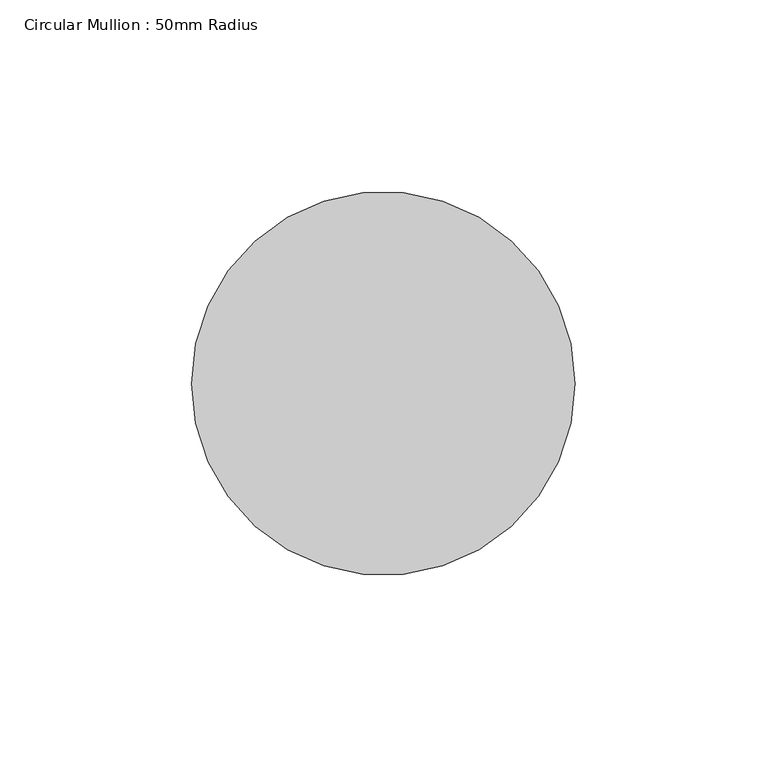
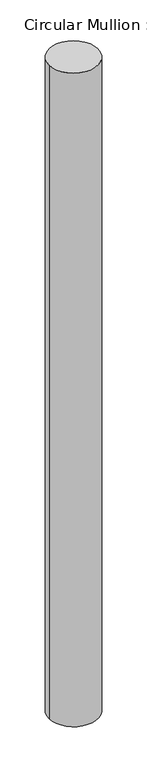
"""IFC4 building model written with IfcOpenShell, lengths in millimetres: member geometry, Circular Mullion : 50mm Radius."""

from ifc_helpers import new_model, si_unit, point, frame, origin, origin_2d, place, context, project, spatial, circle_curve, trimmed, segment, composite_curve, outline, extrude, source, transform, mapped, element, save


def circular_mullion_50mm_radius_f5acd31c(model_context):
    return source(origin(), model_context, "Body", "SweptSolid", [
        extrude(outline(composite_curve([segment(trimmed(circle_curve(origin_2d(), 50.0), [point((50.0, 0.0))], [point((-50.0, 0.0))], False, "CARTESIAN"), True, "CONTINUOUS"), segment(trimmed(circle_curve(origin_2d(), 50.0), [point((-50.0, 0.0))], [point((50.0, 0.0))], False, "CARTESIAN"), True, "CONTINUOUS")], self_intersect=False)), frame((0.0, 0.0, -1414.6605671), z_axis=(0.0, 0.0, 1.0), x_axis=(1.0, 0.0, 0.0)), (0.0, 0.0, 1.0), 1414.6605671),
    ])


if __name__ == "__main__":
    model = new_model("IFC4")
    model_context = context("Model", 3, world=origin())
    ifc_project = project(units=[si_unit("LENGTHUNIT", "METRE", prefix="MILLI")], contexts=[model_context])
    site = spatial("IfcSite", under=ifc_project)
    building = spatial("IfcBuilding", under=site)
    placement = place(None, origin())
    circular_mullion_50mm_radius_shape = circular_mullion_50mm_radius_f5acd31c(model_context)
    element("IfcMember", 1, ObjectType="Circular Mullion : 50mm Radius", at=placement, inside=building, context=model_context, shape_type="MappedRepresentation", body=[
        mapped(circular_mullion_50mm_radius_shape, transform((0.0, 0.0, 0.0), x_axis=(1.0, 0.0, 0.0), y_axis=(0.0, 1.0, 0.0), z_axis=(0.0, 0.0, 1.0))),
    ])
    save(model, "model.ifc")

# Revit data of these elements
# Type "Circular Mullion : 50mm Radius"
#   built-in parameter 1007350 = 0.164042 (stored number, unit not read)
# Element 1 (IfcMember, "Circular Mullion : 50mm Radius")
#   Materials on its faces: "Aluminium"
# Materials
#   "Aluminium": class "Metal", colour RGB 247 247 247, transparency 0, Description = "Aluminium 6061", Cost = 0
